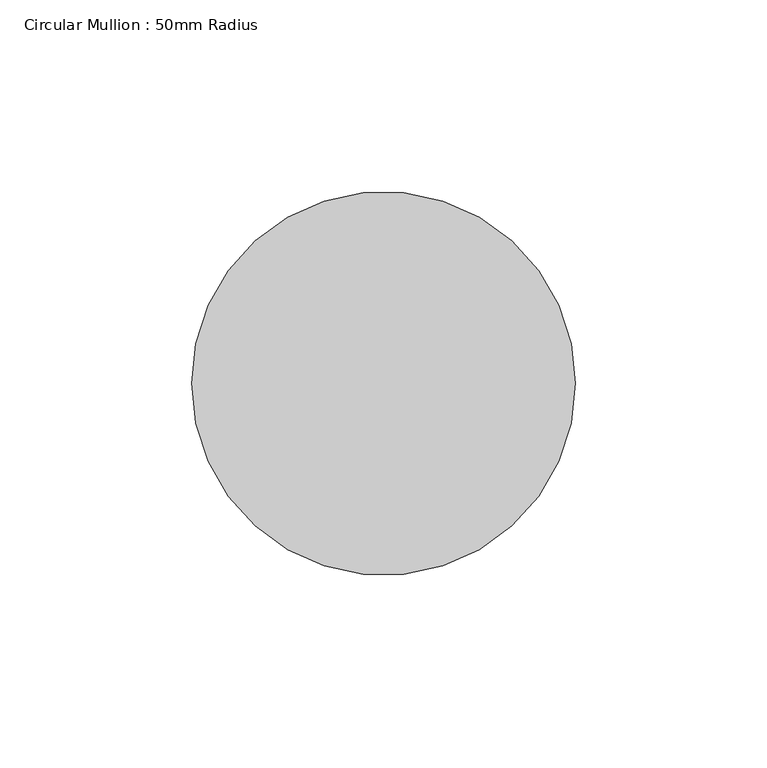
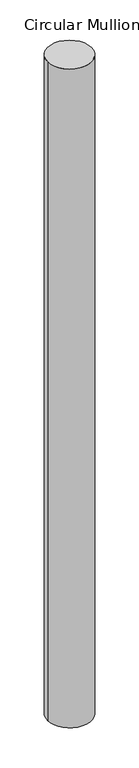
"""IFC4 building model written with IfcOpenShell, lengths in millimetres: member geometry, Circular Mullion : 50mm Radius."""

import ifcopenshell
import ifcopenshell.guid

model = None  # the IFC model being written
_history = None  # IfcOwnerHistory: only IFC2X3 demands one
_inside = {}  # id of a spatial element -> (the spatial element, [elements in it])
_under = {}  # id of a project, library or spatial element -> (it, [spatial elements below it])
_declared = {}  # id of a project -> (the project, [libraries it declares])
_typed = {}  # id of a type object -> (the type object, [elements of that type])
_made_of = {}  # id of a material, layer set ... -> (it, [elements and type objects made of it])


def new_model(schema):
    """Start an empty IFC model of exactly this schema.

    Asked for "IFC4X3", IfcOpenShell would pick the latest addendum, in which some entities
    have other attributes; the version numbers below select the first issue.
    IFC2X3 requires an IfcOwnerHistory on every rooted entity: one is made here for all.
    """
    global model, _history
    if schema == "IFC4X3":
        model = ifcopenshell.file(schema_version=(4, 3, 0, 0))
    else:
        model = ifcopenshell.file(schema=schema)
    _inside.clear()
    _under.clear()
    _declared.clear()
    _typed.clear()
    _made_of.clear()
    _history = None
    if model.schema == "IFC2X3":
        org = make("IfcOrganization", Name="unknown")
        user = make(
            "IfcPersonAndOrganization",
            ThePerson=make("IfcPerson", FamilyName="unknown"),
            TheOrganization=org,
        )
        app = make(
            "IfcApplication",
            ApplicationDeveloper=org,
            Version="unknown",
            ApplicationFullName="unknown",
            ApplicationIdentifier="unknown",
        )
        _history = make(
            "IfcOwnerHistory",
            OwningUser=user,
            OwningApplication=app,
            ChangeAction="ADDED",
            CreationDate=0,
        )
    return model


def make(cls, **values):
    """One entity of the class cls with the attributes given. An attribute that is None is left unset."""
    return model.create_entity(
        cls, **{name: value for name, value in values.items() if value is not None}
    )


def rooted(cls, **values):
    """An entity with a GlobalId (a new one), such as an element, a storey or a relation."""
    return make(cls, GlobalId=ifcopenshell.guid.new(), OwnerHistory=_history, **values)


def si_unit(unit_type, name, prefix=None):
    """IfcSIUnit, for example si_unit("LENGTHUNIT", "METRE", prefix="MILLI")."""
    return make("IfcSIUnit", UnitType=unit_type, Prefix=prefix, Name=name)


def assignment(units):
    """IfcUnitAssignment: the units of a project."""
    return None if units is None else make("IfcUnitAssignment", Units=units)


def point(xyz):
    """IfcCartesianPoint."""
    return None if xyz is None else make("IfcCartesianPoint", Coordinates=xyz)


def direction(xyz):
    """IfcDirection."""
    return None if xyz is None else make("IfcDirection", DirectionRatios=xyz)


def frame(location, z_axis=None, x_axis=None):
    """IfcAxis2Placement3D, a coordinate frame: its origin and axes. An axis left out is left unset."""
    return make(
        "IfcAxis2Placement3D",
        Location=point(location),
        Axis=direction(z_axis),
        RefDirection=direction(x_axis),
    )


def frame_2d(location, x_axis=None):
    """IfcAxis2Placement2D, a coordinate frame in the plane: its origin and x axis."""
    return make(
        "IfcAxis2Placement2D", Location=point(location), RefDirection=direction(x_axis)
    )


def origin():
    """The frame at (0, 0, 0) with its axes left unset."""
    return frame((0.0, 0.0, 0.0))


def origin_2d():
    """The frame at (0, 0) in the plane with its x axis left unset."""
    return frame_2d((0.0, 0.0))


def place(relative_to, where):
    """IfcLocalPlacement: puts the frame where relative to a parent placement (None: the world)."""
    return make(
        "IfcLocalPlacement", PlacementRelTo=relative_to, RelativePlacement=where
    )


def context(
    kind, dimensions, precision=None, world=None, true_north=None, identifier=None
):
    """IfcGeometricRepresentationContext, for example the 3D "Model" context."""
    return make(
        "IfcGeometricRepresentationContext",
        ContextIdentifier=identifier,
        ContextType=kind,
        CoordinateSpaceDimension=dimensions,
        Precision=precision,
        WorldCoordinateSystem=world,
        TrueNorth=true_north,
    )


def project(units=None, contexts=None):
    """IfcProject with its units and contexts."""
    return rooted(
        "IfcProject",
        Name="project",
        RepresentationContexts=contexts,
        UnitsInContext=assignment(units),
    )


def spatial(cls, under=None, at=None, **own):
    """A site, building, storey or space (cls), placed at a placement, below another one or the project."""
    s = rooted(cls, ObjectPlacement=at, **own)
    if under is not None:
        _under.setdefault(under.id(), (under, []))[1].append(s)
    return s


def circle_curve(where, radius):
    """IfcCircle in the frame where."""
    return make("IfcCircle", Position=where, Radius=radius)


def trimmed(basis, trim1, trim2, sense, master):
    """IfcTrimmedCurve: the piece of a basis curve between two trims."""
    return make(
        "IfcTrimmedCurve",
        BasisCurve=basis,
        Trim1=trim1,
        Trim2=trim2,
        SenseAgreement=sense,
        MasterRepresentation=master,
    )


def segment(curve, same_sense, transition):
    """IfcCompositeCurveSegment."""
    return make(
        "IfcCompositeCurveSegment",
        Transition=transition,
        SameSense=same_sense,
        ParentCurve=curve,
    )


def composite_curve(segments, self_intersect=None):
    """IfcCompositeCurve: segments joined end to end."""
    return make("IfcCompositeCurve", Segments=segments, SelfIntersect=self_intersect)


def outline(outer, holes=None, kind="AREA"):
    """IfcArbitraryClosedProfileDef: a profile drawn as a closed curve; with holes, ...WithVoids."""
    if holes is None:
        return make("IfcArbitraryClosedProfileDef", ProfileType=kind, OuterCurve=outer)
    return make(
        "IfcArbitraryProfileDefWithVoids",
        ProfileType=kind,
        OuterCurve=outer,
        InnerCurves=holes,
    )


def extrude(swept, where, along, depth):
    """IfcExtrudedAreaSolid: the profile swept, set in the frame where, extruded along a direction by depth."""
    return make(
        "IfcExtrudedAreaSolid",
        SweptArea=swept,
        Position=where,
        ExtrudedDirection=direction(along),
        Depth=depth,
    )


def shape(context_of_items, identifier, shape_type, items):
    """IfcShapeRepresentation: the items that make up one representation, for example the "Body"."""
    return make(
        "IfcShapeRepresentation",
        ContextOfItems=context_of_items,
        RepresentationIdentifier=identifier,
        RepresentationType=shape_type,
        Items=items,
    )


def source(mapping_origin, context_of_items, identifier, shape_type, items):
    """IfcRepresentationMap: a shape defined once, which mapped items show again and again."""
    return make(
        "IfcRepresentationMap",
        MappingOrigin=mapping_origin,
        MappedRepresentation=shape(context_of_items, identifier, shape_type, items),
    )


def transform(
    local_origin,
    x_axis=None,
    y_axis=None,
    z_axis=None,
    scale=None,
    scale2=None,
    scale3=None,
    uniform=True,
):
    """IfcCartesianTransformationOperator3D, or its non-uniform kind. x_axis, y_axis, z_axis: its Axis1, 2, 3."""
    if uniform:
        return make(
            "IfcCartesianTransformationOperator3D",
            Axis1=direction(x_axis),
            Axis2=direction(y_axis),
            LocalOrigin=point(local_origin),
            Scale=scale,
            Axis3=direction(z_axis),
        )
    return make(
        "IfcCartesianTransformationOperator3DnonUniform",
        Axis1=direction(x_axis),
        Axis2=direction(y_axis),
        LocalOrigin=point(local_origin),
        Scale=scale,
        Axis3=direction(z_axis),
        Scale2=scale2,
        Scale3=scale3,
    )


def mapped(mapping_source, mapping_target):
    """IfcMappedItem: shows the shape of a source again, moved by a transform."""
    return make(
        "IfcMappedItem", MappingSource=mapping_source, MappingTarget=mapping_target
    )


def made_of(thing, what):
    """Note that an element or type object is made of a material, layer set ...; save() writes the relation."""
    if what is not None:
        _made_of.setdefault(what.id(), (what, []))[1].append(thing)
    return thing


def element(
    cls,
    number,
    at=None,
    inside=None,
    cuts=None,
    type_object=None,
    material=None,
    context=None,
    identifier="Body",
    shape_type=None,
    held_by="IfcProductDefinitionShape",
    body=None,
    shapes=None,
    **own,
):
    """One element of the class cls, such as IfcWall. Its Tag is "e" and its number.

    at: its placement. inside: the storey or other place that contains it. cuts: it is an
    opening in that element (IfcRelVoidsElement). A single representation is given by context,
    identifier, shape_type and body (its items); several are given by shapes. held_by: the class
    of the entity that holds the representations. save() writes the other relations.
    """
    e = rooted(cls, Tag="e%d" % number, ObjectPlacement=at, **own)
    if body is not None:
        shapes = [shape(context, identifier, shape_type, body)]
    if shapes is not None:
        e.Representation = make(held_by, Representations=shapes)
    if inside is not None:
        _inside.setdefault(inside.id(), (inside, []))[1].append(e)
    if cuts is not None:
        rooted(
            "IfcRelVoidsElement", RelatingBuildingElement=cuts, RelatedOpeningElement=e
        )
    if type_object is not None:
        _typed.setdefault(type_object.id(), (type_object, []))[1].append(e)
    return made_of(e, material)


def aggregate(whole, parts):
    """IfcRelAggregates: a whole, such as a stair, and the parts it consists of."""
    return rooted("IfcRelAggregates", RelatingObject=whole, RelatedObjects=parts)


def save(model, path):
    """Write the relations noted so far, then the file.

    IfcRelAggregates (storeys below a building ...), IfcRelContainedInSpatialStructure (elements
    in a storey), IfcRelDefinesByType, IfcRelAssociatesMaterial and IfcRelDeclares: one each for
    every whole, place, type object, material and project.
    """
    for whole, parts in _under.values():
        aggregate(whole, parts)
    for where, things in _inside.values():
        rooted(
            "IfcRelContainedInSpatialStructure",
            RelatedElements=things,
            RelatingStructure=where,
        )
    for kind, things in _typed.values():
        rooted("IfcRelDefinesByType", RelatedObjects=things, RelatingType=kind)
    for what, things in _made_of.values():
        rooted("IfcRelAssociatesMaterial", RelatedObjects=things, RelatingMaterial=what)
    for by, libraries in _declared.values():
        rooted("IfcRelDeclares", RelatingContext=by, RelatedDefinitions=libraries)
    model.write(path)


def circular_mullion_50mm_radius_dd1c338a(model_context):
    return source(origin(), model_context, "Body", "SweptSolid", [
        extrude(outline(composite_curve([segment(trimmed(circle_curve(origin_2d(), 50.0), [point((50.0, 0.0))], [point((-50.0, 0.0))], False, "CARTESIAN"), True, "CONTINUOUS"), segment(trimmed(circle_curve(origin_2d(), 50.0), [point((-50.0, 0.0))], [point((50.0, 0.0))], False, "CARTESIAN"), True, "CONTINUOUS")], self_intersect=False)), frame((0.0, 0.0, -1589.0576515), z_axis=(0.0, 0.0, 1.0), x_axis=(1.0, 0.0, 0.0)), (0.0, 0.0, 1.0), 1589.0576515),
    ])


if __name__ == "__main__":
    model = new_model("IFC4")
    model_context = context("Model", 3, world=origin())
    ifc_project = project(units=[si_unit("LENGTHUNIT", "METRE", prefix="MILLI")], contexts=[model_context])
    site = spatial("IfcSite", under=ifc_project)
    building = spatial("IfcBuilding", under=site)
    placement = place(None, origin())
    circular_mullion_50mm_radius_shape = circular_mullion_50mm_radius_dd1c338a(model_context)
    element("IfcMember", 1, ObjectType="Circular Mullion : 50mm Radius", at=placement, inside=building, context=model_context, shape_type="MappedRepresentation", body=[
        mapped(circular_mullion_50mm_radius_shape, transform((0.0, 0.0, 0.0), x_axis=(1.0, 0.0, 0.0), y_axis=(0.0, 1.0, 0.0), z_axis=(0.0, 0.0, 1.0))),
    ])
    save(model, "model.ifc")

# Revit data of these elements
# Type "Circular Mullion : 50mm Radius"
#   built-in parameter 1007350 = 0.164042 (stored number, unit not read)
# Element 1 (IfcMember, "Circular Mullion : 50mm Radius")
#   Materials on its faces: "Aluminium"
# Materials
#   "Aluminium": class "Metal", colour RGB 247 247 247, transparency 0, Description = "Aluminium 6061", Cost = 0
